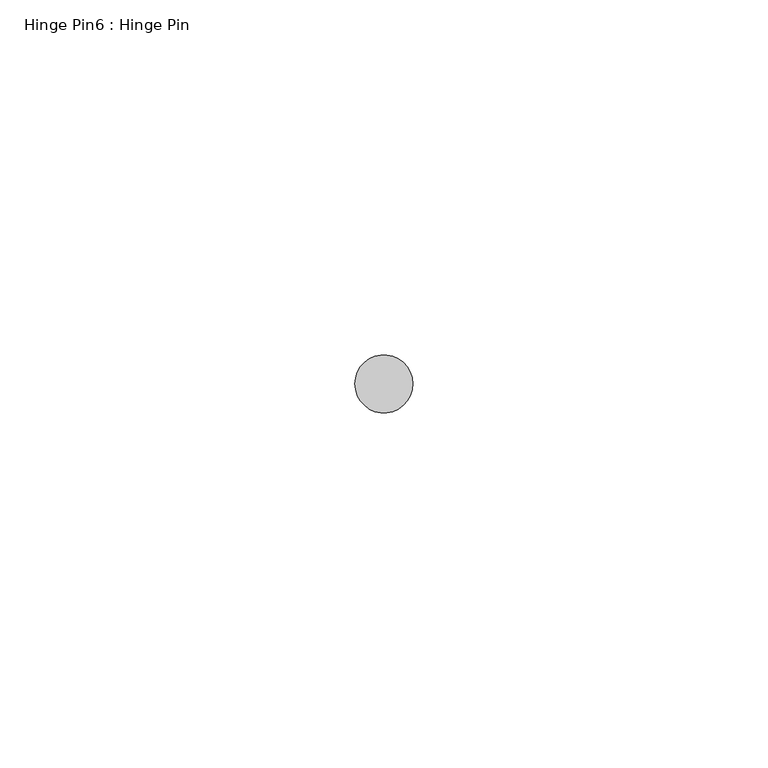
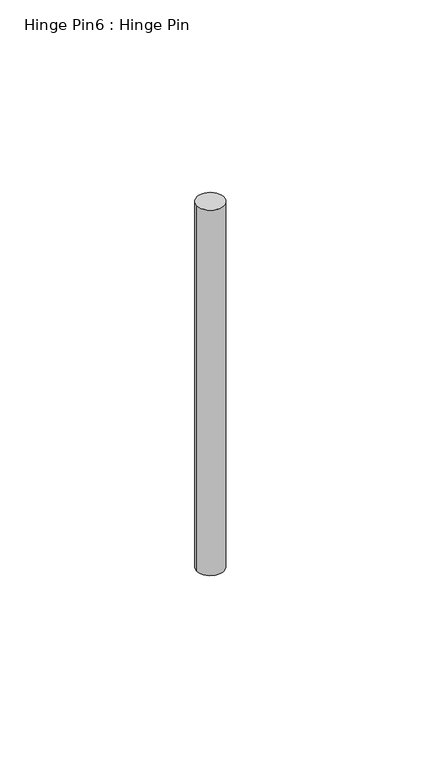
"""IFC4 building model written with IfcOpenShell, lengths in millimetres: proxy geometry, Hinge Pin6 : Hinge Pin."""

from ifc_helpers import new_model, si_unit, point, frame, frame_2d, origin, place, context, project, spatial, circle_curve, trimmed, segment, composite_curve, outline, extrude, source, transform, mapped, element, save


def hinge_pin6_hinge_pin_e1ebbe44(model_context):
    return source(origin(), model_context, "Body", "SweptSolid", [
        extrude(outline(composite_curve([segment(trimmed(circle_curve(frame_2d((587319.1320739, -534100.7049841)), 4.0894), [point((587315.0426739, -534100.7049841))], [point((587323.2214739, -534100.7049841))], False, "CARTESIAN"), True, "CONTINUOUS"), segment(trimmed(circle_curve(frame_2d((587319.1320739, -534100.7049841)), 4.0894), [point((587323.2214739, -534100.7049841))], [point((587315.0426739, -534100.7049841))], False, "CARTESIAN"), True, "CONTINUOUS")], self_intersect=False)), frame((0.0, 0.0, 315.7140625), z_axis=(0.0, 0.0, 1.0), x_axis=(1.0, 0.0, 0.0)), (0.0, 0.0, 1.0), 117.871875),
    ])


if __name__ == "__main__":
    model = new_model("IFC4")
    model_context = context("Model", 3, world=origin())
    ifc_project = project(units=[si_unit("LENGTHUNIT", "METRE", prefix="MILLI")], contexts=[model_context])
    site = spatial("IfcSite", under=ifc_project)
    building = spatial("IfcBuilding", under=site)
    placement = place(None, origin())
    hinge_pin6_hinge_pin_shape = hinge_pin6_hinge_pin_e1ebbe44(model_context)
    element("IfcBuildingElementProxy", 1, Name="Hinge Pin6 : Hinge Pin", ObjectType="Hinge Pin6 : Hinge Pin", at=placement, inside=building, context=model_context, shape_type="MappedRepresentation", body=[
        mapped(hinge_pin6_hinge_pin_shape, transform((0.0, 0.0, 0.0), x_axis=(1.0, 0.0, 0.0), y_axis=(0.0, 1.0, 0.0), z_axis=(0.0, 0.0, 1.0))),
    ])
    save(model, "model.ifc")

# Revit data of these elements
# Element 1 (IfcBuildingElementProxy, "Hinge Pin6 : Hinge Pin")
#   Materials on its faces: "6\"X6\" WELD-ON STL BUTT HINGE"
# Materials
#   "6\"X6\" WELD-ON STL BUTT HINGE": class "Metal", colour RGB 189 187 185, transparency 0, Description = "Carbon steel", Cost = 0
